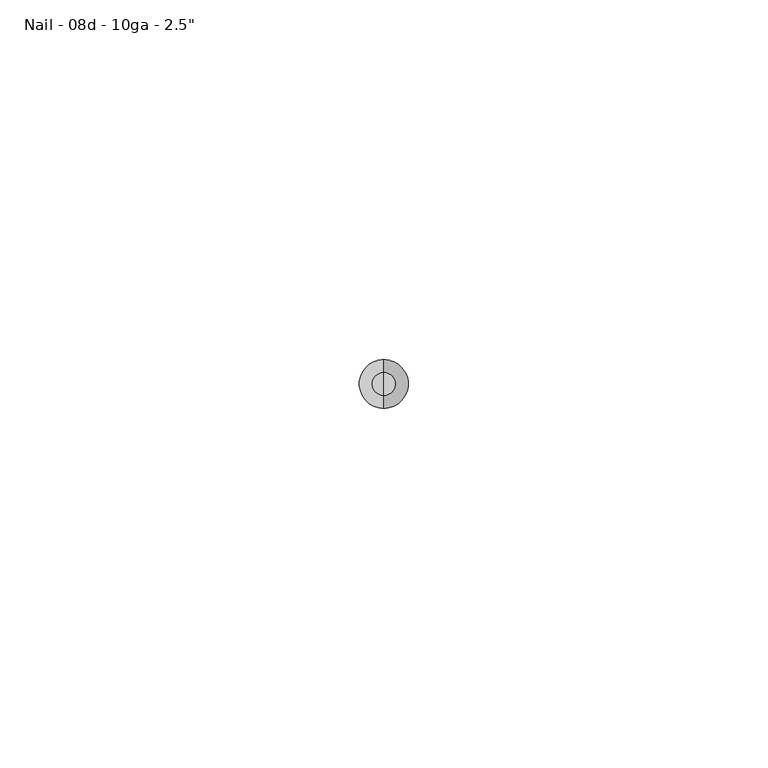
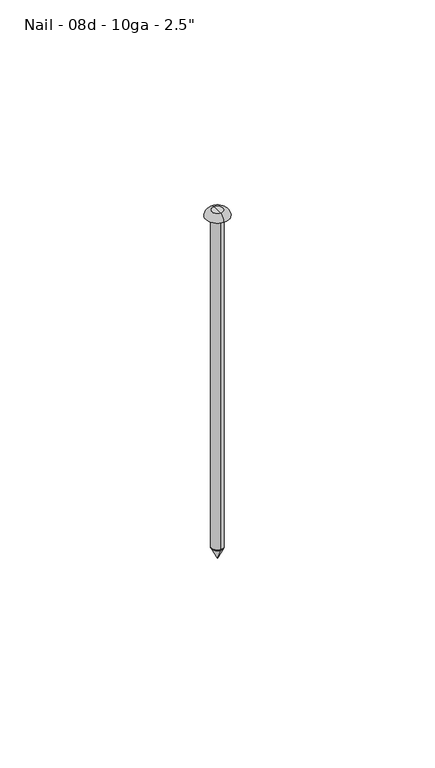
"""IFC4 building model written with IfcOpenShell, lengths in millimetres: fastener geometry."""

from ifc_helpers import new_model, si_unit, point, frame, origin, origin_2d, place, context, project, spatial, polyline, circle_curve, ellipse_curve, trimmed, segment, composite_curve, outline, extrude, source, transform, mapped, element, save
from ifc_brep_helpers import plane_surface, revolved_surface, advanced_brep


def fastener_82244ea5(model_context):
    return source(origin(), model_context, "Body", "SolidModel", [
        advanced_brep(
        [(0.0, -1.7018, -101.6), (0.0, 1.7018, -101.6), (0.0, 0.0, -101.6), (0.0, 0.0, -105.0036)],
        [
            (0, 1, circle_curve(frame((0.0, 0.0, -101.6), z_axis=(0.0, 0.0, 1.0), x_axis=(0.0, 1.0, 0.0)), 1.7018)),
            (1, 2),
            (2, 0),
            (1, 0, circle_curve(frame((0.0, 0.0, -101.6), z_axis=(0.0, 0.0, 1.0), x_axis=(0.0, 1.0, 0.0)), 1.7018)),
            (3, 1),
            (0, 3),
        ],
        [
            plane_surface(frame((0.0, 0.0, -101.6), z_axis=(0.0, 0.0, 1.0), x_axis=(0.0, 1.0, 0.0))),
            revolved_surface(polyline([(0.0, 1.7018, -101.6), (0.0, 0.0, -105.0036)]), (0.0, 0.0, -103.0840259), (0.0, 0.0, -1.0)),
        ],
        [
            (0, [[1, 2, 3]]),
            (0, [[4, -3, -2]]),
            (1, [[5, -1, 6]]),
            (1, [[-6, -4, -5]]),
        ],
    ),
        advanced_brep(
        [(0.0, 3.4036, 0.0), (0.0, -3.4036, 0.0), (0.0, 0.0, 0.0), (0.0, 0.0, 1.7018), (0.0, -1.5875, 1.7018), (0.0, 1.5875, 1.7018)],
        [
            (0, 1, circle_curve(frame((0.0, 0.0, 0.0), z_axis=(0.0, 0.0, -1.0), x_axis=(0.0, -1.0, 0.0)), 3.4036)),
            (1, 2),
            (2, 0),
            (1, 0, circle_curve(frame((0.0, 0.0, 0.0), z_axis=(0.0, 0.0, -1.0), x_axis=(0.0, -1.0, 0.0)), 3.4036)),
            (3, 4),
            (4, 5, circle_curve(frame((0.0, 0.0, 1.7018), z_axis=(0.0, 0.0, 1.0), x_axis=(0.0, -1.0, 0.0)), 1.5875)),
            (5, 3),
            (5, 4, circle_curve(frame((0.0, 0.0, 1.7018), z_axis=(0.0, 0.0, 1.0), x_axis=(0.0, -1.0, 0.0)), 1.5875)),
            (4, 1, circle_curve(frame((0.0, -1.5875, -0.1181384), z_axis=(1.0, 0.0, 0.0), x_axis=(0.0, -1.0, 0.0)), 1.8199384)),
            (0, 5, circle_curve(frame((0.0, 1.5875, -0.1181384), z_axis=(1.0, 0.0, 0.0), x_axis=(0.0, 1.0, 0.0)), 1.8199384)),
        ],
        [
            plane_surface(frame((0.0, 0.0, 0.0), z_axis=(0.0, 0.0, -1.0), x_axis=(0.0, -1.0, 0.0))),
            plane_surface(frame((0.0, 0.0, 1.7018), z_axis=(0.0, 0.0, 1.0), x_axis=(0.0, -1.0, 0.0))),
            revolved_surface(trimmed(ellipse_curve(frame((0.0, -1.5875, -0.1181384), z_axis=(-1.0, 0.0, 0.0), x_axis=(0.0, -1.0, 0.0)), 1.8199384, 1.8199384), [point((0.0, -3.4036, 0.0))], [point((0.0, -1.5875, 1.7018))], True, "CARTESIAN"), (0.0, 0.0, 1.4840259), (0.0, 0.0, 1.0)),
        ],
        [
            (0, [[1, 2, 3]]),
            (0, [[4, -3, -2]]),
            (1, [[5, 6, 7]]),
            (1, [[-7, 8, -5]]),
            (2, [[-6, 9, -1, 10]]),
            (2, [[-8, -10, -4, -9]]),
        ],
    ),
        extrude(outline(composite_curve([segment(trimmed(circle_curve(origin_2d(), 1.7018), [point((0.0, -1.7018))], [point((0.0, 1.7018))], False, "CARTESIAN"), True, "CONTINUOUS"), segment(trimmed(circle_curve(origin_2d(), 1.7018), [point((0.0, 1.7018))], [point((0.0, -1.7018))], False, "CARTESIAN"), True, "CONTINUOUS")], self_intersect=False)), frame((0.0, 0.0, -101.6), z_axis=(0.0, 0.0, 1.0), x_axis=(1.0, 0.0, 0.0)), (0.0, 0.0, 1.0), 101.6),
    ])


if __name__ == "__main__":
    model = new_model("IFC4")
    model_context = context("Model", 3, world=origin())
    ifc_project = project(units=[si_unit("LENGTHUNIT", "METRE", prefix="MILLI")], contexts=[model_context])
    site = spatial("IfcSite", under=ifc_project)
    building = spatial("IfcBuilding", under=site)
    placement = place(None, origin())
    fastener_shape = fastener_82244ea5(model_context)
    element("IfcFastener", 1, ObjectType="060523 - W_P_C - Fastenings - Generic : Nail - 08d - 10ga - 2.5\"", at=placement, inside=building, context=model_context, shape_type="MappedRepresentation", body=[
        mapped(fastener_shape, transform((0.0, 0.0, 0.0), x_axis=(1.0, 0.0, 0.0), y_axis=(0.0, 1.0, 0.0), z_axis=(0.0, 0.0, 1.0))),
    ])
    save(model, "model.ifc")

# Revit data of these elements
# Type "060523 - W_P_C - Fastenings - Generic : Nail - 08d - 10ga - 2.5\""
#   Washer_Thickness = 0' - 0.00333"
#   Washer Radius = 0' - 0.077"
#   Washer Offset - Head = 0' - 0"
#   Washer Offset = 0' - 0"
#   Thickness_of_Substrate [instance default] = 0' - 1"
#   Side = 0' - 0 37/64"
#   Radius = 0' - 0.067"
#   Length [instance default] = 0' - 2 1/2"
#   Head Size = 0' - 1"
#   Head Radius = 0' - 0 1/2"
#   Head Height = 0' - 0.01"
#   Double Diameter = 0' - 0.268"
#   Diameter = 0' - 0.134"
#   Default Elevation = 4' - 0"
#   Washer_Nut_Visibility = no
#   Washer_Head_Visibility = no
#   Round_Head_Visibility = yes
#   Point Visibility = yes
#   Nut_Visibility = no
#   Hex_Head_Visiblilty = no
#   Washer Material = none
#   Bolt Material (Size) = AT SILL - FASTENER AT 24" O.C.
# Element 1 (IfcFastener, "060523 - W_P_C - Fastenings - Generic : Nail - 08d - 10ga - 2.5\"")
#   Length = 0' - 4"
#   Materials on its faces: "AT SILL - FASTENER AT 24\" O.C."
# Materials
#   "AT SILL - FASTENER AT 24\" O.C.": class "Generic", colour RGB 120 120 120, transparency 0, Cost = 0
